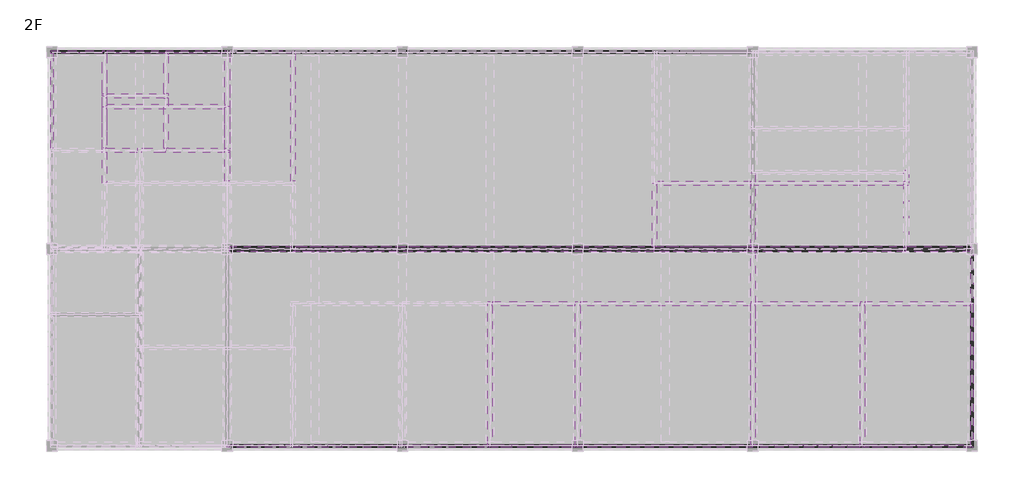
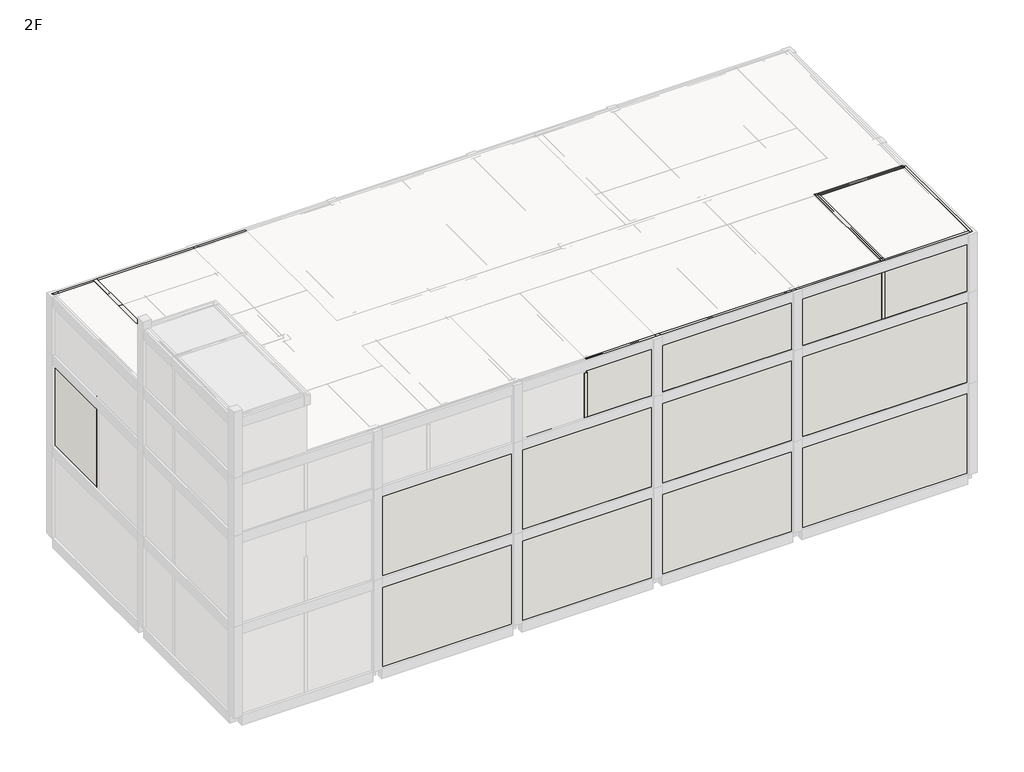
# One storey, part 2 of 7: 53 walls.
"""IFC4 building model written with IfcOpenShell, lengths in millimetres."""

from ifc_helpers import new_model, si_unit, frame, origin, place, context, project, spatial, polyline, outline, extrude, faceted_brep, element, save

model = new_model("IFC4")

# Units and contexts
model_context = context("Model", 3, world=origin())
ifc_project = project(units=[si_unit("LENGTHUNIT", "METRE", prefix="MILLI")], contexts=[model_context])

# Site, building, storey
site = spatial("IfcSite", under=ifc_project)
building = spatial("IfcBuilding", under=site)
storey = spatial("IfcBuildingStorey", under=building, Name="2F", Elevation=3500.0)

# Walls
placement = place(None, origin())
element("IfcWall", 1, ObjectType="WA211_Exterior-Cement Brick-90mm", at=placement, inside=storey, context=model_context, shape_type="Brep", body=[
    faceted_brep([(45402.6521483, 181866.8614395, 3500.0), (45516.6521483, 181866.8614395, 3500.0), (77352.6521483, 181866.8614395, 3500.0), (77352.6521483, 181866.8614395, 9000.0), (45516.6521483, 181866.8614395, 9000.0), (45402.6521483, 181866.8614395, 9000.0), (45402.6521483, 181980.8614395, 3500.0), (45402.6521483, 181980.8614395, 9000.0), (77352.6521483, 181980.8614395, 9000.0), (77352.6521483, 181980.8614395, 3500.0)], [[[0, 1, 2, 3, 4, 5]], [[6, 7, 8, 9]], [[2, 1, 0, 6, 9]], [[5, 4, 3, 8, 7]], [[0, 5, 7, 6]], [[3, 2, 9, 8]]]),
])
element("IfcWall", 2, ObjectType="WA211_Exterior-Cement Brick-90mm", at=placement, inside=storey, context=model_context, shape_type="SweptSolid", body=[
    extrude(outline(polyline([(53566.6521483, 163980.8614395), (87402.6521483, 163980.8614395), (87402.6521483, 163866.8614395), (53566.6521483, 163866.8614395), (53566.6521483, 163980.8614395)])), frame((0.0, 0.0, 3500.0), z_axis=(0.0, 0.0, 1.0), x_axis=(1.0, 0.0, 0.0)), (0.0, 0.0, 1.0), 5500.0),
])
element("IfcWall", 3, ObjectType="WA211_Exterior-Cement Brick-90mm", at=placement, inside=storey, context=model_context, shape_type="Brep", body=[
    faceted_brep([(87402.6521483, 172923.8614395, 3500.0), (87402.6521483, 172816.8614395, 3500.0), (87402.6521483, 163980.8614395, 3500.0), (87402.6521483, 163866.8614395, 3500.0), (87402.6521483, 163866.8614395, 9000.0), (87402.6521483, 163980.8614395, 9000.0), (87402.6521483, 172816.8614395, 9000.0), (87402.6521483, 172923.8614395, 9000.0), (87516.6521483, 172923.8614395, 3500.0), (87516.6521483, 172923.8614395, 9000.0), (87516.6521483, 163866.8614395, 9000.0), (87516.6521483, 163866.8614395, 3500.0)], [[[0, 1, 2, 3, 4, 5, 6, 7]], [[8, 9, 10, 11]], [[3, 2, 1, 0, 8, 11]], [[7, 6, 5, 4, 10, 9]], [[0, 7, 9, 8]], [[4, 3, 11, 10]]]),
])
element("IfcWall", 4, ObjectType="WA211_Exterior-Cement Brick-90mm", at=placement, inside=storey, context=model_context, shape_type="Brep", body=[
    faceted_brep([(77459.6521483, 163980.8614395, 9000.0), (77352.6521483, 163980.8614395, 9000.0), (53566.6521483, 163980.8614395, 9000.0), (53566.6521483, 163980.8614395, 12000.0), (53459.6521483, 163980.8614395, 12000.0), (53459.6521483, 163980.8614395, 14500.0), (77352.6521483, 163980.8614395, 14500.0), (77459.6521483, 163980.8614395, 14500.0), (77459.6521483, 163866.8614395, 9000.0), (77459.6521483, 163866.8614395, 14500.0), (53459.6521483, 163866.8614395, 14500.0), (53459.6521483, 163866.8614395, 12000.0), (53566.6521483, 163866.8614395, 12000.0), (53566.6521483, 163866.8614395, 9000.0)], [[[0, 1, 2, 3, 4, 5, 6, 7]], [[8, 9, 10, 11, 12, 13]], [[2, 1, 0, 8, 13]], [[7, 6, 5, 10, 9]], [[0, 7, 9, 8]], [[5, 4, 11, 10]], [[11, 4, 3, 12]], [[3, 2, 13, 12]]]),
])
element("IfcWall", 5, ObjectType="WA211_Exterior-Cement Brick-90mm", at=placement, inside=storey, context=model_context, shape_type="Brep", body=[
    faceted_brep([(87402.6521483, 163980.8614395, 9000.0), (77566.6521483, 163980.8614395, 9000.0), (77459.6521483, 163980.8614395, 9000.0), (77459.6521483, 163980.8614395, 14500.0), (77566.6521483, 163980.8614395, 14500.0), (87402.6521483, 163980.8614395, 14500.0), (87402.6521483, 163866.8614395, 9000.0), (87402.6521483, 163866.8614395, 14500.0), (77459.6521483, 163866.8614395, 14500.0), (77459.6521483, 163866.8614395, 9000.0)], [[[0, 1, 2, 3, 4, 5]], [[6, 7, 8, 9]], [[2, 1, 0, 6, 9]], [[3, 2, 9, 8]], [[5, 4, 3, 8, 7]], [[0, 5, 7, 6]]]),
])
element("IfcWall", 6, ObjectType="WA211_Exterior-Cement Brick-90mm", at=placement, inside=storey, context=model_context, shape_type="Brep", body=[
    faceted_brep([(87402.6521483, 172923.8614395, 9000.0), (87402.6521483, 172816.8614395, 9000.0), (87402.6521483, 163980.8614395, 9000.0), (87402.6521483, 163866.8614395, 9000.0), (87402.6521483, 163866.8614395, 14500.0), (87402.6521483, 163980.8614395, 14500.0), (87402.6521483, 172816.8614395, 14500.0), (87402.6521483, 172923.8614395, 14500.0), (87516.6521483, 172923.8614395, 9000.0), (87516.6521483, 172923.8614395, 14500.0), (87516.6521483, 163866.8614395, 14500.0), (87516.6521483, 163866.8614395, 9000.0)], [[[0, 1, 2, 3, 4, 5, 6, 7]], [[8, 9, 10, 11]], [[3, 2, 1, 0, 8, 11]], [[7, 6, 5, 4, 10, 9]], [[0, 7, 9, 8]], [[4, 3, 11, 10]]]),
])
element("IfcWall", 7, ObjectType="WA211_Exterior-Cement Brick-90mm", at=placement, inside=storey, context=model_context, shape_type="SweptSolid", body=[
    extrude(outline(polyline([(45516.6521483, 181866.8614395), (45516.6521483, 177530.8614395), (45402.6521483, 177530.8614395), (45402.6521483, 181866.8614395), (45516.6521483, 181866.8614395)])), frame((0.0, 0.0, 9000.0), z_axis=(0.0, 0.0, 1.0), x_axis=(1.0, 0.0, 0.0)), (0.0, 0.0, 1.0), 5500.0),
])
element("IfcWall", 8, ObjectType="WA211_Exterior-Cement Brick-90mm", at=placement, inside=storey, context=model_context, shape_type="Brep", body=[
    faceted_brep([(45402.6521483, 181866.8614395, 9000.0), (45516.6521483, 181866.8614395, 9000.0), (47752.6521483, 181866.8614395, 9000.0), (47752.6521483, 181866.8614395, 14500.0), (45516.6521483, 181866.8614395, 14500.0), (45402.6521483, 181866.8614395, 14500.0), (45402.6521483, 181980.8614395, 9000.0), (45402.6521483, 181980.8614395, 14500.0), (47752.6521483, 181980.8614395, 14500.0), (47752.6521483, 181980.8614395, 9000.0)], [[[0, 1, 2, 3, 4, 5]], [[6, 7, 8, 9]], [[2, 1, 0, 6, 9]], [[5, 4, 3, 8, 7]], [[0, 5, 7, 6]], [[3, 2, 9, 8]]]),
])
element("IfcWall", 9, ObjectType="WA211_Exterior-Cement Brick-90mm", at=placement, inside=storey, context=model_context, shape_type="Brep", body=[
    faceted_brep([(50659.6521483, 181866.8614395, 14500.0), (50659.6521483, 181866.8614395, 9000.0), (50766.6521483, 181866.8614395, 9000.0), (53352.6521483, 181866.8614395, 9000.0), (53352.6521483, 181866.8614395, 12400.0), (53459.6521483, 181866.8614395, 12400.0), (53459.6521483, 181866.8614395, 14500.0), (50659.6521483, 181980.8614395, 9000.0), (50659.6521483, 181980.8614395, 14500.0), (53459.6521483, 181980.8614395, 14500.0), (53459.6521483, 181980.8614395, 12400.0), (53352.6521483, 181980.8614395, 12400.0), (53352.6521483, 181980.8614395, 9000.0)], [[[0, 1, 2, 3, 4, 5, 6]], [[7, 8, 9, 10, 11, 12]], [[3, 2, 1, 7, 12]], [[0, 6, 9, 8]], [[6, 5, 10, 9]], [[10, 5, 4, 11]], [[4, 3, 12, 11]], [[0, 8, 7, 1]]]),
])
element("IfcWall", 10, ObjectType="WA211_Exterior-Cement Brick-90mm", at=placement, inside=storey, context=model_context, shape_type="Brep", body=[
    faceted_brep([(47966.6521483, 181866.8614395, 9000.0), (50552.6521483, 181866.8614395, 9000.0), (50659.6521483, 181866.8614395, 9000.0), (50659.6521483, 181866.8614395, 14500.0), (47966.6521483, 181866.8614395, 14500.0), (47966.6521483, 181980.8614395, 9000.0), (47966.6521483, 181980.8614395, 14500.0), (50659.6521483, 181980.8614395, 14500.0), (50659.6521483, 181980.8614395, 9000.0)], [[[0, 1, 2, 3, 4]], [[5, 6, 7, 8]], [[2, 1, 0, 5, 8]], [[4, 3, 7, 6]], [[0, 4, 6, 5]], [[2, 8, 7, 3]]]),
])
element("IfcWall", 11, ObjectType="WA211_Exterior-Cement Brick-90mm", at=placement, inside=storey, context=model_context, shape_type="SweptSolid", body=[
    extrude(outline(polyline([(14500.0, 69352.6521483), (17200.0, 69352.6521483), (17200.0, 69459.6521483), (18000.0, 69459.6521483), (18000.0, 65459.6521483), (17200.0, 65459.6521483), (17200.0, 65566.6521483), (14500.0, 65566.6521483), (14500.0, 69352.6521483)])), frame((0.0, 163866.8614395, 0.0), z_axis=(0.0, 1.0, 0.0), x_axis=(0.0, 0.0, 1.0)), (0.0, 0.0, 1.0), 114.0),
])
element("IfcWall", 12, ObjectType="WA211_Exterior-Cement Brick-90mm", at=placement, inside=storey, context=model_context, shape_type="Brep", body=[
    faceted_brep([(77459.6521483, 163980.8614395, 18000.0), (77459.6521483, 163980.8614395, 14500.0), (77352.6521483, 163980.8614395, 14500.0), (69566.6521483, 163980.8614395, 14500.0), (69566.6521483, 163980.8614395, 17200.0), (69459.6521483, 163980.8614395, 17200.0), (69459.6521483, 163980.8614395, 18000.0), (77459.6521483, 163866.8614395, 14500.0), (77459.6521483, 163866.8614395, 18000.0), (69459.6521483, 163866.8614395, 18000.0), (69459.6521483, 163866.8614395, 17200.0), (69566.6521483, 163866.8614395, 17200.0), (69566.6521483, 163866.8614395, 14500.0)], [[[0, 1, 2, 3, 4, 5, 6]], [[7, 8, 9, 10, 11, 12]], [[3, 2, 1, 7, 12]], [[0, 6, 9, 8]], [[6, 5, 10, 9]], [[10, 5, 4, 11]], [[4, 3, 12, 11]], [[0, 8, 7, 1]]]),
])
element("IfcWall", 13, ObjectType="WA211_Exterior-Cement Brick-90mm", at=placement, inside=storey, context=model_context, shape_type="Brep", body=[
    faceted_brep([(82352.6521483, 163980.8614395, 14500.0), (77566.6521483, 163980.8614395, 14500.0), (77459.6521483, 163980.8614395, 14500.0), (77459.6521483, 163980.8614395, 18000.0), (82352.6521483, 163980.8614395, 18000.0), (82352.6521483, 163866.8614395, 14500.0), (82352.6521483, 163866.8614395, 18000.0), (77459.6521483, 163866.8614395, 18000.0), (77459.6521483, 163866.8614395, 14500.0)], [[[0, 1, 2, 3, 4]], [[5, 6, 7, 8]], [[2, 1, 0, 5, 8]], [[4, 3, 7, 6]], [[2, 8, 7, 3]], [[0, 4, 6, 5]]]),
])
element("IfcWall", 14, ObjectType="WA211_Exterior-Cement Brick-90mm", at=placement, inside=storey, context=model_context, shape_type="SweptSolid", body=[
    extrude(outline(polyline([(82566.6521483, 163980.8614395), (87402.6521483, 163980.8614395), (87402.6521483, 163866.8614395), (82566.6521483, 163866.8614395), (82566.6521483, 163980.8614395)])), frame((0.0, 0.0, 14500.0), z_axis=(0.0, 0.0, 1.0), x_axis=(1.0, 0.0, 0.0)), (0.0, 0.0, 1.0), 3500.0),
])
element("IfcWall", 15, ObjectType="WA211_Exterior-Cement Brick-90mm", at=placement, inside=storey, context=model_context, shape_type="Brep", body=[
    faceted_brep([(87402.6521483, 170423.8614395, 14500.0), (87402.6521483, 170316.8614395, 14500.0), (87402.6521483, 163980.8614395, 14500.0), (87402.6521483, 163866.8614395, 14500.0), (87402.6521483, 163866.8614395, 18000.0), (87402.6521483, 163980.8614395, 18000.0), (87402.6521483, 170316.8614395, 18000.0), (87402.6521483, 170423.8614395, 18000.0), (87516.6521483, 170423.8614395, 14500.0), (87516.6521483, 170423.8614395, 18000.0), (87516.6521483, 163866.8614395, 18000.0), (87516.6521483, 163866.8614395, 14500.0)], [[[0, 1, 2, 3, 4, 5, 6, 7]], [[8, 9, 10, 11]], [[3, 2, 1, 0, 8, 11]], [[7, 6, 5, 4, 10, 9]], [[0, 7, 9, 8]], [[4, 3, 11, 10]]]),
])
element("IfcWall", 16, ObjectType="WA211_Exterior-Cement Brick-90mm", at=placement, inside=storey, context=model_context, shape_type="SweptSolid", body=[
    extrude(outline(polyline([(14500.0, 47966.6521483), (14500.0, 53352.6521483), (17200.0, 53352.6521483), (17200.0, 53459.6521483), (18000.0, 53459.6521483), (18000.0, 47966.6521483), (14500.0, 47966.6521483)])), frame((0.0, 181866.8614395, 0.0), z_axis=(0.0, 1.0, 0.0), x_axis=(0.0, 0.0, 1.0)), (0.0, 0.0, 1.0), 114.0),
])
element("IfcWall", 17, ObjectType="WA211_Exterior-Cement Brick-90mm", at=placement, inside=storey, context=model_context, shape_type="SweptSolid", body=[
    extrude(outline(polyline([(14500.0, 53566.6521483), (14500.0, 56352.6521483), (17200.0, 56352.6521483), (17200.0, 56459.6521483), (18000.0, 56459.6521483), (18000.0, 53459.6521483), (17200.0, 53459.6521483), (17200.0, 53566.6521483), (14500.0, 53566.6521483)])), frame((0.0, 181866.8614395, 0.0), z_axis=(0.0, 1.0, 0.0), x_axis=(0.0, 0.0, 1.0)), (0.0, 0.0, 1.0), 114.0),
])
element("IfcWall", 18, ObjectType="WA211_Exterior-Cement Brick-90mm", at=placement, inside=storey, context=model_context, shape_type="Brep", body=[
    faceted_brep([(45402.6521483, 181866.8614395, 14500.0), (45516.6521483, 181866.8614395, 14500.0), (47752.6521483, 181866.8614395, 14500.0), (47752.6521483, 181866.8614395, 18000.0), (45516.6521483, 181866.8614395, 18000.0), (45402.6521483, 181866.8614395, 18000.0), (45402.6521483, 181980.8614395, 14500.0), (45402.6521483, 181980.8614395, 18000.0), (47752.6521483, 181980.8614395, 18000.0), (47752.6521483, 181980.8614395, 14500.0)], [[[0, 1, 2, 3, 4, 5]], [[6, 7, 8, 9]], [[2, 1, 0, 6, 9]], [[5, 4, 3, 8, 7]], [[3, 2, 9, 8]], [[0, 5, 7, 6]]]),
])
element("IfcWall", 19, ObjectType="WA221_Interior-Cement Block-190mm", at=placement, inside=storey, context=model_context, shape_type="SweptSolid", body=[
    extrude(outline(polyline([(53566.6521483, 173030.8614395), (77352.6521483, 173030.8614395), (77352.6521483, 172816.8614395), (53566.6521483, 172816.8614395), (53566.6521483, 173030.8614395)])), frame((0.0, 0.0, 3500.0), z_axis=(0.0, 0.0, 1.0), x_axis=(1.0, 0.0, 0.0)), (0.0, 0.0, 1.0), 5500.0),
])
element("IfcWall", 20, ObjectType="WA221_Interior-Cement Block-190mm", at=placement, inside=storey, context=model_context, shape_type="Brep", body=[
    faceted_brep([(77566.6521483, 172816.8614395, 3500.0), (87402.6521483, 172816.8614395, 3500.0), (87402.6521483, 172816.8614395, 9000.0), (77566.6521483, 172816.8614395, 9000.0), (77566.6521483, 173030.8614395, 3500.0), (77566.6521483, 173030.8614395, 9000.0), (87402.6521483, 173030.8614395, 9000.0), (87402.6521483, 173030.8614395, 3500.0), (87402.6521483, 172923.8614395, 3500.0), (87402.6521483, 172923.8614395, 9000.0)], [[[0, 1, 2, 3]], [[4, 5, 6, 7]], [[1, 0, 4, 7, 8]], [[3, 2, 9, 6, 5]], [[0, 3, 5, 4]], [[2, 1, 8, 7, 6, 9]]]),
])
element("IfcWall", 21, ObjectType="WA221_Interior-Cement Block-190mm", at=placement, inside=storey, context=model_context, shape_type="Brep", body=[
    faceted_brep([(77459.6521483, 173030.8614395, 9000.0), (77352.6521483, 173030.8614395, 9000.0), (53566.6521483, 173030.8614395, 9000.0), (53566.6521483, 173030.8614395, 12400.0), (77352.6521483, 173030.8614395, 12400.0), (77459.6521483, 173030.8614395, 12400.0), (77459.6521483, 172816.8614395, 9000.0), (77459.6521483, 172816.8614395, 12400.0), (77352.6521483, 172816.8614395, 12400.0), (53566.6521483, 172816.8614395, 12400.0), (53566.6521483, 172816.8614395, 12000.0), (53566.6521483, 172816.8614395, 9000.0), (77352.6521483, 172816.8614395, 9000.0), (53566.6521483, 172923.8614395, 9000.0)], [[[0, 1, 2, 3, 4, 5]], [[6, 7, 8, 9, 10, 11, 12]], [[2, 1, 0, 6, 12, 11, 13]], [[5, 4, 3, 9, 8, 7]], [[0, 5, 7, 6]], [[2, 13, 11, 10, 9, 3]]]),
])
element("IfcWall", 22, ObjectType="WA221_Interior-Cement Block-190mm", at=placement, inside=storey, context=model_context, shape_type="Brep", body=[
    faceted_brep([(77352.6521483, 176316.8614395, 9000.0), (77352.6521483, 173030.8614395, 9000.0), (77352.6521483, 173030.8614395, 12400.0), (77352.6521483, 176423.8614395, 12400.0), (77352.6521483, 176423.8614395, 11700.0), (77352.6521483, 176316.8614395, 11700.0), (77566.6521483, 176316.8614395, 9000.0), (77566.6521483, 176316.8614395, 11700.0), (77566.6521483, 176423.8614395, 11700.0), (77566.6521483, 176423.8614395, 12400.0), (77566.6521483, 173030.8614395, 12400.0), (77566.6521483, 173030.8614395, 9000.0), (77459.6521483, 173030.8614395, 9000.0), (77459.6521483, 173030.8614395, 12400.0)], [[[0, 1, 2, 3, 4, 5]], [[6, 7, 8, 9, 10, 11]], [[1, 0, 6, 11, 12]], [[3, 2, 13, 10, 9]], [[2, 1, 12, 11, 10, 13]], [[4, 3, 9, 8]], [[4, 8, 7, 5]], [[0, 5, 7, 6]]]),
])
element("IfcWall", 23, ObjectType="WA221_Interior-Cement Block-190mm", at=placement, inside=storey, context=model_context, shape_type="Brep", body=[
    faceted_brep([(53566.6521483, 177530.8614395, 9000.0), (53566.6521483, 181866.8614395, 9000.0), (53566.6521483, 181980.8614395, 9000.0), (53566.6521483, 181980.8614395, 12400.0), (53566.6521483, 181866.8614395, 12400.0), (53566.6521483, 177423.8614395, 12400.0), (53566.6521483, 177423.8614395, 11700.0), (53566.6521483, 177530.8614395, 11700.0), (53352.6521483, 177530.8614395, 9000.0), (53352.6521483, 177530.8614395, 11700.0), (53352.6521483, 177423.8614395, 11700.0), (53352.6521483, 177423.8614395, 12400.0), (53352.6521483, 181866.8614395, 12400.0), (53352.6521483, 181980.8614395, 12400.0), (53352.6521483, 181980.8614395, 9000.0), (53352.6521483, 181866.8614395, 9000.0), (53459.6521483, 181980.8614395, 12400.0)], [[[0, 1, 2, 3, 4, 5, 6, 7]], [[8, 9, 10, 11, 12, 13, 14, 15]], [[2, 1, 0, 8, 15, 14]], [[5, 4, 3, 16, 13, 12, 11]], [[3, 2, 14, 13, 16]], [[6, 5, 11, 10]], [[6, 10, 9, 7]], [[0, 7, 9, 8]]]),
])
element("IfcWall", 24, ObjectType="WA221_Interior-Cement Block-190mm", at=placement, inside=storey, context=model_context, shape_type="Brep", body=[
    faceted_brep([(77566.6521483, 163980.8614395, 9000.0), (77566.6521483, 172816.8614395, 9000.0), (77566.6521483, 172816.8614395, 14500.0), (77566.6521483, 163980.8614395, 14500.0), (77352.6521483, 163980.8614395, 9000.0), (77352.6521483, 163980.8614395, 14500.0), (77352.6521483, 172816.8614395, 14500.0), (77352.6521483, 172816.8614395, 12400.0), (77352.6521483, 172816.8614395, 9000.0), (77459.6521483, 163980.8614395, 9000.0), (77459.6521483, 172816.8614395, 9000.0), (77459.6521483, 163980.8614395, 14500.0)], [[[0, 1, 2, 3]], [[4, 5, 6, 7, 8]], [[1, 0, 9, 4, 8, 10]], [[3, 2, 6, 5, 11]], [[1, 10, 8, 7, 6, 2]], [[0, 3, 11, 5, 4, 9]]]),
])
element("IfcWall", 25, ObjectType="WA221_Interior-Cement Block-190mm", at=placement, inside=storey, context=model_context, shape_type="Brep", body=[
    faceted_brep([(77459.6521483, 172816.8614395, 9000.0), (77566.6521483, 172816.8614395, 9000.0), (84459.6521483, 172816.8614395, 9000.0), (84459.6521483, 172816.8614395, 14500.0), (77566.6521483, 172816.8614395, 14500.0), (77352.6521483, 172816.8614395, 14500.0), (77352.6521483, 172816.8614395, 12400.0), (77459.6521483, 172816.8614395, 12400.0), (77459.6521483, 173030.8614395, 9000.0), (77459.6521483, 173030.8614395, 12400.0), (77352.6521483, 173030.8614395, 12400.0), (77352.6521483, 173030.8614395, 14500.0), (84459.6521483, 173030.8614395, 14500.0), (84459.6521483, 173030.8614395, 9000.0), (84352.6521483, 173030.8614395, 9000.0), (77566.6521483, 173030.8614395, 9000.0)], [[[0, 1, 2, 3, 4, 5, 6, 7]], [[8, 9, 10, 11, 12, 13, 14, 15]], [[2, 1, 0, 8, 15, 14, 13]], [[5, 4, 3, 12, 11]], [[0, 7, 9, 8]], [[6, 10, 9, 7]], [[6, 5, 11, 10]], [[2, 13, 12, 3]]]),
])
element("IfcWall", 26, ObjectType="WA221_Interior-Cement Block-190mm", at=placement, inside=storey, context=model_context, shape_type="Brep", body=[
    faceted_brep([(84459.6521483, 172816.8614395, 14500.0), (84459.6521483, 172816.8614395, 9000.0), (87402.6521483, 172816.8614395, 9000.0), (87402.6521483, 172816.8614395, 14500.0), (84459.6521483, 173030.8614395, 9000.0), (84459.6521483, 173030.8614395, 14500.0), (87402.6521483, 173030.8614395, 14500.0), (87402.6521483, 173030.8614395, 9000.0), (84566.6521483, 173030.8614395, 9000.0), (87402.6521483, 172923.8614395, 9000.0), (87402.6521483, 172923.8614395, 14500.0)], [[[0, 1, 2, 3]], [[4, 5, 6, 7, 8]], [[2, 1, 4, 8, 7, 9]], [[0, 3, 10, 6, 5]], [[3, 2, 9, 7, 6, 10]], [[0, 5, 4, 1]]]),
])
element("IfcWall", 27, ObjectType="WA221_Interior-Cement Block-190mm", at=placement, inside=storey, context=model_context, shape_type="Brep", body=[
    faceted_brep([(84352.6521483, 176530.8614395, 9000.0), (84352.6521483, 176316.8614395, 9000.0), (84352.6521483, 173030.8614395, 9000.0), (84352.6521483, 173030.8614395, 11700.0), (84352.6521483, 176316.8614395, 11700.0), (84352.6521483, 176530.8614395, 11700.0), (84566.6521483, 176530.8614395, 9000.0), (84566.6521483, 176530.8614395, 11700.0), (84566.6521483, 173030.8614395, 11700.0), (84566.6521483, 173030.8614395, 9000.0), (84459.6521483, 173030.8614395, 9000.0)], [[[0, 1, 2, 3, 4, 5]], [[6, 7, 8, 9]], [[2, 1, 0, 6, 9, 10]], [[5, 4, 3, 8, 7]], [[0, 5, 7, 6]], [[3, 2, 10, 9, 8]]]),
])
element("IfcWall", 28, ObjectType="WA221_Interior-Cement Block-190mm", at=placement, inside=storey, context=model_context, shape_type="Brep", body=[
    faceted_brep([(47752.6521483, 181980.8614395, 9000.0), (47752.6521483, 181866.8614395, 9000.0), (47752.6521483, 180030.8614395, 9000.0), (47752.6521483, 180030.8614395, 11700.0), (47752.6521483, 179923.8614395, 11700.0), (47752.6521483, 179923.8614395, 14500.0), (47752.6521483, 181866.8614395, 14500.0), (47752.6521483, 181980.8614395, 14500.0), (47966.6521483, 181980.8614395, 9000.0), (47966.6521483, 181980.8614395, 14500.0), (47966.6521483, 181866.8614395, 14500.0), (47966.6521483, 179923.8614395, 14500.0), (47966.6521483, 179923.8614395, 11700.0), (47966.6521483, 180030.8614395, 11700.0), (47966.6521483, 180030.8614395, 9000.0), (47966.6521483, 181866.8614395, 9000.0)], [[[0, 1, 2, 3, 4, 5, 6, 7]], [[8, 9, 10, 11, 12, 13, 14, 15]], [[2, 1, 0, 8, 15, 14]], [[7, 6, 5, 11, 10, 9]], [[0, 7, 9, 8]], [[5, 4, 12, 11]], [[12, 4, 3, 13]], [[3, 2, 14, 13]]]),
])
element("IfcWall", 29, ObjectType="WA221_Interior-Cement Block-190mm", at=placement, inside=storey, context=model_context, shape_type="Brep", body=[
    faceted_brep([(47752.6521483, 179816.8614395, 9000.0), (47752.6521483, 177530.8614395, 9000.0), (47752.6521483, 177530.8614395, 14500.0), (47752.6521483, 179923.8614395, 14500.0), (47752.6521483, 179923.8614395, 11700.0), (47752.6521483, 179816.8614395, 11700.0), (47966.6521483, 179816.8614395, 9000.0), (47966.6521483, 179816.8614395, 11700.0), (47966.6521483, 179923.8614395, 11700.0), (47966.6521483, 179923.8614395, 14500.0), (47966.6521483, 177530.8614395, 14500.0), (47966.6521483, 177530.8614395, 11700.0), (47966.6521483, 177530.8614395, 9000.0), (47859.6521483, 177530.8614395, 9000.0)], [[[0, 1, 2, 3, 4, 5]], [[6, 7, 8, 9, 10, 11, 12]], [[1, 0, 6, 12, 13]], [[3, 2, 10, 9]], [[1, 13, 12, 11, 10, 2]], [[4, 3, 9, 8]], [[4, 8, 7, 5]], [[0, 5, 7, 6]]]),
])
element("IfcWall", 30, ObjectType="WA221_Interior-Cement Block-190mm", at=placement, inside=storey, context=model_context, shape_type="Brep", body=[
    faceted_brep([(49352.6521483, 177530.8614395, 9000.0), (47966.6521483, 177530.8614395, 9000.0), (47859.6521483, 177530.8614395, 9000.0), (47859.6521483, 177530.8614395, 11700.0), (47966.6521483, 177530.8614395, 11700.0), (49352.6521483, 177530.8614395, 11700.0), (49352.6521483, 177316.8614395, 9000.0), (49352.6521483, 177316.8614395, 11700.0), (47966.6521483, 177316.8614395, 11700.0), (47859.6521483, 177316.8614395, 11700.0), (47859.6521483, 177316.8614395, 9000.0)], [[[0, 1, 2, 3, 4, 5]], [[6, 7, 8, 9, 10]], [[2, 1, 0, 6, 10]], [[3, 2, 10, 9]], [[5, 4, 3, 9, 8, 7]], [[0, 5, 7, 6]]]),
])
element("IfcWall", 31, ObjectType="WA221_Interior-Cement Block-190mm", at=placement, inside=storey, context=model_context, shape_type="Brep", body=[
    faceted_brep([(50552.6521483, 181866.8614395, 9000.0), (50552.6521483, 180030.8614395, 9000.0), (50552.6521483, 180030.8614395, 11700.0), (50552.6521483, 181866.8614395, 11700.0), (50766.6521483, 181866.8614395, 9000.0), (50766.6521483, 181866.8614395, 11700.0), (50766.6521483, 180030.8614395, 11700.0), (50766.6521483, 180030.8614395, 9000.0), (50659.6521483, 181866.8614395, 9000.0)], [[[0, 1, 2, 3]], [[4, 5, 6, 7]], [[1, 0, 8, 4, 7]], [[3, 2, 6, 5]], [[0, 3, 5, 4, 8]], [[2, 1, 7, 6]]]),
])
element("IfcWall", 32, ObjectType="WA221_Interior-Cement Block-190mm", at=placement, inside=storey, context=model_context, shape_type="Brep", body=[
    faceted_brep([(50766.6521483, 177530.8614395, 9000.0), (50766.6521483, 179816.8614395, 9000.0), (50766.6521483, 179816.8614395, 11700.0), (50766.6521483, 177530.8614395, 11700.0), (50552.6521483, 177530.8614395, 9000.0), (50552.6521483, 177530.8614395, 11700.0), (50552.6521483, 179816.8614395, 11700.0), (50552.6521483, 179816.8614395, 9000.0), (50659.6521483, 177530.8614395, 9000.0), (50659.6521483, 177530.8614395, 11700.0)], [[[0, 1, 2, 3]], [[4, 5, 6, 7]], [[1, 0, 8, 4, 7]], [[3, 2, 6, 5, 9]], [[0, 3, 9, 5, 4, 8]], [[2, 1, 7, 6]]]),
])
element("IfcWall", 33, ObjectType="WA221_Interior-Cement Block-190mm", at=placement, inside=storey, context=model_context, shape_type="Brep", body=[
    faceted_brep([(50659.6521483, 177316.8614395, 9000.0), (53352.6521483, 177316.8614395, 9000.0), (53566.6521483, 177316.8614395, 9000.0), (53566.6521483, 177316.8614395, 11700.0), (53352.6521483, 177316.8614395, 11700.0), (50659.6521483, 177316.8614395, 11700.0), (50659.6521483, 177530.8614395, 9000.0), (50659.6521483, 177530.8614395, 11700.0), (50766.6521483, 177530.8614395, 11700.0), (53352.6521483, 177530.8614395, 11700.0), (53566.6521483, 177530.8614395, 11700.0), (53566.6521483, 177530.8614395, 9000.0), (53352.6521483, 177530.8614395, 9000.0), (50766.6521483, 177530.8614395, 9000.0), (53566.6521483, 177423.8614395, 11700.0)], [[[0, 1, 2, 3, 4, 5]], [[6, 7, 8, 9, 10, 11, 12, 13]], [[2, 1, 0, 6, 13, 12, 11]], [[5, 4, 3, 14, 10, 9, 8, 7]], [[0, 5, 7, 6]], [[3, 2, 11, 10, 14]]]),
])
element("IfcWall", 34, ObjectType="WA221_Interior-Cement Block-190mm", at=placement, inside=storey, context=model_context, shape_type="Brep", body=[
    faceted_brep([(50766.6521483, 180030.8614395, 9000.0), (50552.6521483, 180030.8614395, 9000.0), (47966.6521483, 180030.8614395, 9000.0), (47752.6521483, 180030.8614395, 9000.0), (47752.6521483, 180030.8614395, 11700.0), (47966.6521483, 180030.8614395, 11700.0), (50552.6521483, 180030.8614395, 11700.0), (50766.6521483, 180030.8614395, 11700.0), (50766.6521483, 179816.8614395, 9000.0), (50766.6521483, 179816.8614395, 11700.0), (50552.6521483, 179816.8614395, 11700.0), (47966.6521483, 179816.8614395, 11700.0), (47752.6521483, 179816.8614395, 11700.0), (47752.6521483, 179816.8614395, 9000.0), (47966.6521483, 179816.8614395, 9000.0), (50552.6521483, 179816.8614395, 9000.0), (47752.6521483, 179923.8614395, 11700.0)], [[[0, 1, 2, 3, 4, 5, 6, 7]], [[8, 9, 10, 11, 12, 13, 14, 15]], [[3, 2, 1, 0, 8, 15, 14, 13]], [[7, 6, 5, 4, 16, 12, 11, 10, 9]], [[0, 7, 9, 8]], [[4, 3, 13, 12, 16]]]),
])
element("IfcWall", 35, ObjectType="WA221_Interior-Cement Block-190mm", at=placement, inside=storey, context=model_context, shape_type="Brep", body=[
    faceted_brep([(50659.6521483, 177530.8614395, 9000.0), (50552.6521483, 177530.8614395, 9000.0), (49566.6521483, 177530.8614395, 9000.0), (49566.6521483, 177530.8614395, 11700.0), (50552.6521483, 177530.8614395, 11700.0), (50659.6521483, 177530.8614395, 11700.0), (50659.6521483, 177316.8614395, 9000.0), (50659.6521483, 177316.8614395, 11700.0), (49566.6521483, 177316.8614395, 11700.0), (49566.6521483, 177316.8614395, 9000.0)], [[[0, 1, 2, 3, 4, 5]], [[6, 7, 8, 9]], [[2, 1, 0, 6, 9]], [[5, 4, 3, 8, 7]], [[0, 5, 7, 6]], [[3, 2, 9, 8]]]),
])
element("IfcWall", 36, ObjectType="WA221_Interior-Cement Block-190mm", at=placement, inside=storey, context=model_context, shape_type="Brep", body=[
    faceted_brep([(65352.6521483, 170530.8614395, 14500.0), (65352.6521483, 170316.8614395, 14500.0), (65352.6521483, 163980.8614395, 14500.0), (65352.6521483, 163866.8614395, 14500.0), (65352.6521483, 163866.8614395, 17200.0), (65352.6521483, 163980.8614395, 17200.0), (65352.6521483, 170316.8614395, 17200.0), (65352.6521483, 170530.8614395, 17200.0), (65566.6521483, 170530.8614395, 14500.0), (65566.6521483, 170530.8614395, 17200.0), (65566.6521483, 170316.8614395, 17200.0), (65566.6521483, 163980.8614395, 17200.0), (65566.6521483, 163866.8614395, 17200.0), (65566.6521483, 163866.8614395, 14500.0), (65566.6521483, 163980.8614395, 14500.0), (65566.6521483, 170316.8614395, 14500.0), (65459.6521483, 163866.8614395, 17200.0)], [[[0, 1, 2, 3, 4, 5, 6, 7]], [[8, 9, 10, 11, 12, 13, 14, 15]], [[3, 2, 1, 0, 8, 15, 14, 13]], [[7, 6, 5, 4, 16, 12, 11, 10, 9]], [[4, 3, 13, 12, 16]], [[0, 7, 9, 8]]]),
])
element("IfcWall", 37, ObjectType="WA221_Interior-Cement Block-190mm", at=placement, inside=storey, context=model_context, shape_type="Brep", body=[
    faceted_brep([(69566.6521483, 163866.8614395, 14500.0), (69566.6521483, 163980.8614395, 14500.0), (69566.6521483, 170316.8614395, 14500.0), (69566.6521483, 170530.8614395, 14500.0), (69566.6521483, 170530.8614395, 17200.0), (69566.6521483, 170316.8614395, 17200.0), (69566.6521483, 163980.8614395, 17200.0), (69566.6521483, 163866.8614395, 17200.0), (69352.6521483, 163866.8614395, 14500.0), (69352.6521483, 163866.8614395, 17200.0), (69352.6521483, 163980.8614395, 17200.0), (69352.6521483, 170316.8614395, 17200.0), (69352.6521483, 170530.8614395, 17200.0), (69352.6521483, 170530.8614395, 14500.0), (69352.6521483, 170316.8614395, 14500.0), (69352.6521483, 163980.8614395, 14500.0), (69459.6521483, 163866.8614395, 17200.0)], [[[0, 1, 2, 3, 4, 5, 6, 7]], [[8, 9, 10, 11, 12, 13, 14, 15]], [[3, 2, 1, 0, 8, 15, 14, 13]], [[7, 6, 5, 4, 12, 11, 10, 9, 16]], [[4, 3, 13, 12]], [[0, 7, 16, 9, 8]]]),
])
element("IfcWall", 38, ObjectType="WA221_Interior-Cement Block-190mm", at=placement, inside=storey, context=model_context, shape_type="SweptSolid", body=[
    extrude(outline(polyline([(65566.6521483, 170530.8614395), (69352.6521483, 170530.8614395), (69352.6521483, 170316.8614395), (65566.6521483, 170316.8614395), (65566.6521483, 170530.8614395)])), frame((0.0, 0.0, 14500.0), z_axis=(0.0, 0.0, 1.0), x_axis=(1.0, 0.0, 0.0)), (0.0, 0.0, 1.0), 2700.0),
])
element("IfcWall", 39, ObjectType="WA221_Interior-Cement Block-190mm", at=placement, inside=storey, context=model_context, shape_type="Brep", body=[
    faceted_brep([(84566.6521483, 176030.8614395, 14500.0), (84352.6521483, 176030.8614395, 14500.0), (73066.6521483, 176030.8614395, 14500.0), (73066.6521483, 176030.8614395, 17200.0), (84352.6521483, 176030.8614395, 17200.0), (84566.6521483, 176030.8614395, 17200.0), (84566.6521483, 175816.8614395, 14500.0), (84566.6521483, 175816.8614395, 17200.0), (84352.6521483, 175816.8614395, 17200.0), (73066.6521483, 175816.8614395, 17200.0), (73066.6521483, 175816.8614395, 14500.0), (84352.6521483, 175816.8614395, 14500.0), (73066.6521483, 175923.8614395, 14500.0), (73066.6521483, 175923.8614395, 17200.0)], [[[0, 1, 2, 3, 4, 5]], [[6, 7, 8, 9, 10, 11]], [[2, 1, 0, 6, 11, 10, 12]], [[5, 4, 3, 13, 9, 8, 7]], [[0, 5, 7, 6]], [[3, 2, 12, 10, 9, 13]]]),
])
element("IfcWall", 40, ObjectType="WA221_Interior-Cement Block-190mm", at=placement, inside=storey, context=model_context, shape_type="Brep", body=[
    faceted_brep([(77352.6521483, 170530.8614395, 14500.0), (77352.6521483, 170316.8614395, 14500.0), (77352.6521483, 163980.8614395, 14500.0), (77352.6521483, 163980.8614395, 17200.0), (77352.6521483, 170316.8614395, 17200.0), (77352.6521483, 170530.8614395, 17200.0), (77566.6521483, 170530.8614395, 14500.0), (77566.6521483, 170530.8614395, 17200.0), (77566.6521483, 170316.8614395, 17200.0), (77566.6521483, 163980.8614395, 17200.0), (77566.6521483, 163980.8614395, 14500.0), (77566.6521483, 170316.8614395, 14500.0), (77459.6521483, 163980.8614395, 14500.0)], [[[0, 1, 2, 3, 4, 5]], [[6, 7, 8, 9, 10, 11]], [[2, 1, 0, 6, 11, 10, 12]], [[5, 4, 3, 9, 8, 7]], [[0, 5, 7, 6]], [[3, 2, 12, 10, 9]]]),
])
element("IfcWall", 41, ObjectType="WA221_Interior-Cement Block-190mm", at=placement, inside=storey, context=model_context, shape_type="SweptSolid", body=[
    extrude(outline(polyline([(77352.6521483, 170316.8614395), (69566.6521483, 170316.8614395), (69566.6521483, 170530.8614395), (77352.6521483, 170530.8614395), (77352.6521483, 170316.8614395)])), frame((0.0, 0.0, 14500.0), z_axis=(0.0, 0.0, 1.0), x_axis=(1.0, 0.0, 0.0)), (0.0, 0.0, 1.0), 2700.0),
])
element("IfcWall", 42, ObjectType="WA221_Interior-Cement Block-190mm", at=placement, inside=storey, context=model_context, shape_type="Brep", body=[
    faceted_brep([(73066.6521483, 173030.8614395, 14500.0), (73066.6521483, 175816.8614395, 14500.0), (73066.6521483, 175923.8614395, 14500.0), (73066.6521483, 175923.8614395, 17200.0), (73066.6521483, 175816.8614395, 17200.0), (73066.6521483, 173030.8614395, 17200.0), (72852.6521483, 173030.8614395, 14500.0), (72852.6521483, 173030.8614395, 17200.0), (72852.6521483, 175923.8614395, 17200.0), (72852.6521483, 175923.8614395, 14500.0), (72959.6521483, 173030.8614395, 14500.0), (72959.6521483, 173030.8614395, 17200.0)], [[[0, 1, 2, 3, 4, 5]], [[6, 7, 8, 9]], [[2, 1, 0, 10, 6, 9]], [[3, 2, 9, 8]], [[5, 4, 3, 8, 7, 11]], [[0, 5, 11, 7, 6, 10]]]),
])
element("IfcWall", 43, ObjectType="WA221_Interior-Cement Block-190mm", at=placement, inside=storey, context=model_context, shape_type="Brep", body=[
    faceted_brep([(56352.6521483, 181980.8614395, 14500.0), (56352.6521483, 181866.8614395, 14500.0), (56352.6521483, 176030.8614395, 14500.0), (56352.6521483, 176030.8614395, 17200.0), (56352.6521483, 181866.8614395, 17200.0), (56352.6521483, 181980.8614395, 17200.0), (56566.6521483, 181980.8614395, 14500.0), (56566.6521483, 181980.8614395, 17200.0), (56566.6521483, 181866.8614395, 17200.0), (56566.6521483, 176030.8614395, 17200.0), (56566.6521483, 176030.8614395, 14500.0), (56566.6521483, 181866.8614395, 14500.0), (56459.6521483, 181980.8614395, 17200.0)], [[[0, 1, 2, 3, 4, 5]], [[6, 7, 8, 9, 10, 11]], [[2, 1, 0, 6, 11, 10]], [[5, 4, 3, 9, 8, 7, 12]], [[0, 5, 12, 7, 6]], [[3, 2, 10, 9]]]),
])
element("IfcWall", 44, ObjectType="WA221_Interior-Cement Block-190mm", at=placement, inside=storey, context=model_context, shape_type="Brep", body=[
    faceted_brep([(72959.6521483, 173030.8614395, 14500.0), (72852.6521483, 173030.8614395, 14500.0), (56566.6521483, 173030.8614395, 14500.0), (56566.6521483, 173030.8614395, 17200.0), (72852.6521483, 173030.8614395, 17200.0), (72959.6521483, 173030.8614395, 17200.0), (72959.6521483, 172816.8614395, 14500.0), (72959.6521483, 172816.8614395, 17200.0), (56566.6521483, 172816.8614395, 17200.0), (56566.6521483, 172816.8614395, 14500.0)], [[[0, 1, 2, 3, 4, 5]], [[6, 7, 8, 9]], [[2, 1, 0, 6, 9]], [[5, 4, 3, 8, 7]], [[0, 5, 7, 6]], [[3, 2, 9, 8]]]),
])
element("IfcWall", 45, ObjectType="WA221_Interior-Cement Block-190mm", at=placement, inside=storey, context=model_context, shape_type="Brep", body=[
    faceted_brep([(82566.6521483, 163866.8614395, 14500.0), (82566.6521483, 163980.8614395, 14500.0), (82566.6521483, 170316.8614395, 14500.0), (82566.6521483, 170530.8614395, 14500.0), (82566.6521483, 170530.8614395, 18000.0), (82566.6521483, 170316.8614395, 18000.0), (82566.6521483, 163980.8614395, 18000.0), (82566.6521483, 163866.8614395, 18000.0), (82352.6521483, 163866.8614395, 14500.0), (82352.6521483, 163866.8614395, 18000.0), (82352.6521483, 163980.8614395, 18000.0), (82352.6521483, 170530.8614395, 18000.0), (82352.6521483, 170530.8614395, 17200.0), (82352.6521483, 170530.8614395, 14500.0), (82352.6521483, 170316.8614395, 14500.0), (82352.6521483, 163980.8614395, 14500.0)], [[[0, 1, 2, 3, 4, 5, 6, 7]], [[8, 9, 10, 11, 12, 13, 14, 15]], [[3, 2, 1, 0, 8, 15, 14, 13]], [[7, 6, 5, 4, 11, 10, 9]], [[3, 13, 12, 11, 4]], [[0, 7, 9, 8]]]),
])
element("IfcWall", 46, ObjectType="WA221_Interior-Cement Block-190mm", at=placement, inside=storey, context=model_context, shape_type="SweptSolid", body=[
    extrude(outline(polyline([(82352.6521483, 170316.8614395), (77566.6521483, 170316.8614395), (77566.6521483, 170530.8614395), (82352.6521483, 170530.8614395), (82352.6521483, 170316.8614395)])), frame((0.0, 0.0, 14500.0), z_axis=(0.0, 0.0, 1.0), x_axis=(1.0, 0.0, 0.0)), (0.0, 0.0, 1.0), 2700.0),
])
element("IfcWall", 47, ObjectType="WA221_Interior-Cement Block-190mm", at=placement, inside=storey, context=model_context, shape_type="Brep", body=[
    faceted_brep([(82566.6521483, 170316.8614395, 14500.0), (87402.6521483, 170316.8614395, 14500.0), (87402.6521483, 170316.8614395, 18000.0), (82566.6521483, 170316.8614395, 18000.0), (82566.6521483, 170530.8614395, 14500.0), (82566.6521483, 170530.8614395, 18000.0), (87402.6521483, 170530.8614395, 18000.0), (87402.6521483, 170530.8614395, 14500.0), (87402.6521483, 170423.8614395, 14500.0), (87402.6521483, 170423.8614395, 18000.0)], [[[0, 1, 2, 3]], [[4, 5, 6, 7]], [[1, 0, 4, 7, 8]], [[3, 2, 9, 6, 5]], [[0, 3, 5, 4]], [[2, 1, 8, 7, 6, 9]]]),
])
element("IfcWall", 48, ObjectType="WA221_Interior-Cement Block-190mm", at=placement, inside=storey, context=model_context, shape_type="Brep", body=[
    faceted_brep([(84352.6521483, 173030.8614395, 14500.0), (73066.6521483, 173030.8614395, 14500.0), (72959.6521483, 173030.8614395, 14500.0), (72959.6521483, 173030.8614395, 17200.0), (73066.6521483, 173030.8614395, 17200.0), (84352.6521483, 173030.8614395, 17200.0), (84352.6521483, 172816.8614395, 14500.0), (84352.6521483, 172816.8614395, 17200.0), (72959.6521483, 172816.8614395, 17200.0), (72959.6521483, 172816.8614395, 14500.0)], [[[0, 1, 2, 3, 4, 5]], [[6, 7, 8, 9]], [[2, 1, 0, 6, 9]], [[3, 2, 9, 8]], [[5, 4, 3, 8, 7]], [[0, 5, 7, 6]]]),
])
element("IfcWall", 49, ObjectType="WA221_Interior-Cement Block-190mm", at=placement, inside=storey, context=model_context, shape_type="Brep", body=[
    faceted_brep([(53352.6521483, 179530.8614395, 14500.0), (47966.6521483, 179530.8614395, 14500.0), (47966.6521483, 179530.8614395, 17200.0), (53352.6521483, 179530.8614395, 17200.0), (53352.6521483, 179316.8614395, 14500.0), (53352.6521483, 179316.8614395, 17200.0), (47966.6521483, 179316.8614395, 17200.0), (47966.6521483, 179316.8614395, 14500.0), (53352.6521483, 179423.8614395, 14500.0), (47966.6521483, 179423.8614395, 14500.0), (53352.6521483, 179423.8614395, 17200.0)], [[[0, 1, 2, 3]], [[4, 5, 6, 7]], [[1, 0, 8, 4, 7, 9]], [[3, 2, 6, 5, 10]], [[0, 3, 10, 5, 4, 8]], [[2, 1, 9, 7, 6]]]),
])
element("IfcWall", 50, ObjectType="WA221_Interior-Cement Block-190mm", at=placement, inside=storey, context=model_context, shape_type="Brep", body=[
    faceted_brep([(53352.6521483, 179423.8614395, 14500.0), (53352.6521483, 179316.8614395, 14500.0), (53352.6521483, 176030.8614395, 14500.0), (53352.6521483, 176030.8614395, 17200.0), (53352.6521483, 179316.8614395, 17200.0), (53352.6521483, 179423.8614395, 17200.0), (53566.6521483, 179423.8614395, 14500.0), (53566.6521483, 179423.8614395, 17200.0), (53566.6521483, 176030.8614395, 17200.0), (53566.6521483, 176030.8614395, 14500.0), (53459.6521483, 176030.8614395, 14500.0), (53459.6521483, 176030.8614395, 17200.0)], [[[0, 1, 2, 3, 4, 5]], [[6, 7, 8, 9]], [[2, 1, 0, 6, 9, 10]], [[5, 4, 3, 11, 8, 7]], [[0, 5, 7, 6]], [[3, 2, 10, 9, 8, 11]]]),
])
element("IfcWall", 51, ObjectType="WA221_Interior-Cement Block-190mm", at=placement, inside=storey, context=model_context, shape_type="Brep", body=[
    faceted_brep([(47752.6521483, 179423.8614395, 18000.0), (47752.6521483, 179423.8614395, 14500.0), (47752.6521483, 175923.8614395, 14500.0), (47752.6521483, 175923.8614395, 18000.0), (47966.6521483, 179423.8614395, 14500.0), (47966.6521483, 179423.8614395, 18000.0), (47966.6521483, 175923.8614395, 18000.0), (47966.6521483, 175923.8614395, 14500.0), (47966.6521483, 176030.8614395, 14500.0), (47966.6521483, 179316.8614395, 14500.0)], [[[0, 1, 2, 3]], [[4, 5, 6, 7, 8, 9]], [[2, 1, 4, 9, 8, 7]], [[0, 3, 6, 5]], [[0, 5, 4, 1]], [[2, 7, 6, 3]]]),
])
element("IfcWall", 52, ObjectType="WA221_Interior-Cement Block-190mm", at=placement, inside=storey, context=model_context, shape_type="Brep", body=[
    faceted_brep([(53352.6521483, 181980.8614395, 14500.0), (53352.6521483, 181866.8614395, 14500.0), (53352.6521483, 179530.8614395, 14500.0), (53352.6521483, 179423.8614395, 14500.0), (53352.6521483, 179423.8614395, 17200.0), (53352.6521483, 179530.8614395, 17200.0), (53352.6521483, 181866.8614395, 17200.0), (53352.6521483, 181980.8614395, 17200.0), (53566.6521483, 181980.8614395, 14500.0), (53566.6521483, 181980.8614395, 17200.0), (53566.6521483, 181866.8614395, 17200.0), (53566.6521483, 179423.8614395, 17200.0), (53566.6521483, 179423.8614395, 14500.0), (53566.6521483, 181866.8614395, 14500.0), (53459.6521483, 181980.8614395, 17200.0)], [[[0, 1, 2, 3, 4, 5, 6, 7]], [[8, 9, 10, 11, 12, 13]], [[3, 2, 1, 0, 8, 13, 12]], [[4, 3, 12, 11]], [[7, 6, 5, 4, 11, 10, 9, 14]], [[0, 7, 14, 9, 8]]]),
])
element("IfcWall", 53, ObjectType="WA221_Interior-Cement Block-190mm", at=placement, inside=storey, context=model_context, shape_type="Brep", body=[
    faceted_brep([(47752.6521483, 181980.8614395, 14500.0), (47752.6521483, 181866.8614395, 14500.0), (47752.6521483, 179423.8614395, 14500.0), (47752.6521483, 179423.8614395, 18000.0), (47752.6521483, 181866.8614395, 18000.0), (47752.6521483, 181980.8614395, 18000.0), (47966.6521483, 181980.8614395, 14500.0), (47966.6521483, 181980.8614395, 18000.0), (47966.6521483, 181866.8614395, 18000.0), (47966.6521483, 179423.8614395, 18000.0), (47966.6521483, 179423.8614395, 14500.0), (47966.6521483, 179530.8614395, 14500.0), (47966.6521483, 181866.8614395, 14500.0)], [[[0, 1, 2, 3, 4, 5]], [[6, 7, 8, 9, 10, 11, 12]], [[2, 1, 0, 6, 12, 11, 10]], [[5, 4, 3, 9, 8, 7]], [[2, 10, 9, 3]], [[0, 5, 7, 6]]]),
])

save(model, "model.ifc")

# Revit data of these elements
# Type "WA211_Exterior-Cement Brick-90mm"
#   Type Comments = ""
#   Layers, outside or top first: 0 mm "A04AL081-00001_Skirt_Acrylic Emulsion Paint" (function 100); 0 mm "A04AL077-00001_Ext Wall Painting_Acrylic Emulsion Paint" (function 100); 12 mm "A04AS164-00001_Plastering_Ext" (function 4); 90 mm "A04AK073-00001_Concrete Brick_0.5B" (function 1); 12 mm "A04AS164-00002_Plastering_Int" (function 5); 0 mm "A04AL078-00002_Int Wall Painting_Water Emulsion Paint" (function 100); 0 mm "A04AL081-00001_Skirt_Acrylic Emulsion Paint" (function 100)
# Type "WA221_Interior-Cement Block-190mm"
#   Type Comments = ""
#   Layers, outside or top first: 0 mm "A04AL081-00001_Skirt_Acrylic Emulsion Paint" (function 100); 0 mm "A04AL078-00002_Int Wall Painting_Water Emulsion Paint" (function 100); 12 mm "A04AS164-00002_Plastering_Int" (function 2); 190 mm "A04AK069-00002_Reinforced Concrete Block_THK 100-200mm" (function 1); 12 mm "A04AS164-00002_Plastering_Int" (function 2); 0 mm "A04AL078-00002_Int Wall Painting_Water Emulsion Paint" (function 100); 0 mm "A04AL081-00001_Skirt_Acrylic Emulsion Paint" (function 100)
# Elements 1, 3 (IfcWall, "WA211_Exterior-Cement Brick-90mm")
#   Top Offset = 0 mm
#   Base Offset = 0 mm
#   Unconnected Height = 5500 mm
#   wall height = 5500 mm
#   Phase Created = New Construction
#   Base Constraint = 2F
#   Materials on its faces: "Default Wall", "A04AS164-00001_Plastering_Ext", "A04AS164-00002_Plastering_Int"
# Element 2 (IfcWall, "WA211_Exterior-Cement Brick-90mm")
#   Top Offset = 0 mm
#   Base Offset = 0 mm
#   Unconnected Height = 5500 mm
#   wall height = 5500 mm
#   Phase Created = New Construction
#   Base Constraint = 2F
#   Materials on its faces: "Default Wall", "A04AS164-00002_Plastering_Int", "A04AS164-00001_Plastering_Ext"
# Elements 4, 5, 7, 9, 10 (IfcWall, "WA211_Exterior-Cement Brick-90mm")
#   Top Offset = 0 mm
#   Base Offset = 0 mm
#   Unconnected Height = 5500 mm
#   wall height = 5500 mm
#   Phase Created = New Construction
#   Base Constraint = 3F
#   Materials on its faces: "Default Wall", "A04AS164-00002_Plastering_Int", "A04AS164-00001_Plastering_Ext"
# Elements 6, 8 (IfcWall, "WA211_Exterior-Cement Brick-90mm")
#   Top Offset = 0 mm
#   Base Offset = 0 mm
#   Unconnected Height = 5500 mm
#   wall height = 5500 mm
#   Phase Created = New Construction
#   Base Constraint = 3F
#   Materials on its faces: "Default Wall", "A04AS164-00001_Plastering_Ext", "A04AS164-00002_Plastering_Int"
# Elements 11, 12, 13, 14, 16, 17 (IfcWall, "WA211_Exterior-Cement Brick-90mm")
#   Top Offset = 0 mm
#   Base Offset = 0 mm
#   Unconnected Height = 3500 mm
#   wall height = 3500 mm
#   Phase Created = New Construction
#   Base Constraint = 4F
#   Materials on its faces: "Default Wall", "A04AS164-00002_Plastering_Int", "A04AS164-00001_Plastering_Ext"
# Elements 15, 18 (IfcWall, "WA211_Exterior-Cement Brick-90mm")
#   Top Offset = 0 mm
#   Base Offset = 0 mm
#   Unconnected Height = 3500 mm
#   wall height = 3500 mm
#   Phase Created = New Construction
#   Base Constraint = 4F
#   Materials on its faces: "Default Wall", "A04AS164-00001_Plastering_Ext", "A04AS164-00002_Plastering_Int"
# Elements 19, 20 (IfcWall, "WA221_Interior-Cement Block-190mm")
#   Top Offset = 0 mm
#   Base Offset = 0 mm
#   Unconnected Height = 5500 mm
#   wall height = 5500 mm
#   Phase Created = New Construction
#   Base Constraint = 2F
#   Materials on its faces: "Default Wall", "A04AS164-00002_Plastering_Int"
# Elements 21, 22 (IfcWall, "WA221_Interior-Cement Block-190mm")
#   Top Offset = 0 mm
#   Base Offset = 0 mm
#   Unconnected Height = 3400 mm
#   wall height = 3400 mm
#   Phase Created = New Construction
#   Base Constraint = 3F
#   Materials on its faces: "Default Wall", "A04AS164-00002_Plastering_Int"
# Element 23 (IfcWall, "WA221_Interior-Cement Block-190mm")
#   Top Offset = 0 mm
#   Base Offset = 0 mm
#   Unconnected Height = 3400 mm
#   wall height = 3400 mm
#   Phase Created = New Construction
#   Base Constraint = 3F
#   Materials on its faces: "Default Wall", "A04AS164-00002_Plastering_Int", "A04AS164-00001_Plastering_Ext"
# Elements 24, 25, 26, 29 (IfcWall, "WA221_Interior-Cement Block-190mm")
#   Top Offset = 0 mm
#   Base Offset = 0 mm
#   Unconnected Height = 5500 mm
#   wall height = 5500 mm
#   Phase Created = New Construction
#   Base Constraint = 3F
#   Materials on its faces: "Default Wall", "A04AS164-00002_Plastering_Int"
# Elements 27, 33, 34 (IfcWall, "WA221_Interior-Cement Block-190mm")
#   Top Offset = 0 mm
#   Base Offset = 0 mm
#   Unconnected Height = 2700 mm
#   wall height = 2700 mm
#   Phase Created = New Construction
#   Base Constraint = 3F
#   Materials on its faces: "A04AS164-00002_Plastering_Int", "Default Wall"
# Element 28 (IfcWall, "WA221_Interior-Cement Block-190mm")
#   Top Offset = 0 mm
#   Base Offset = 0 mm
#   Unconnected Height = 5500 mm
#   wall height = 5500 mm
#   Phase Created = New Construction
#   Base Constraint = 3F
#   Materials on its faces: "Default Wall", "A04AS164-00002_Plastering_Int", "A04AS164-00001_Plastering_Ext"
# Elements 30, 31, 32, 35 (IfcWall, "WA221_Interior-Cement Block-190mm")
#   Top Offset = 0 mm
#   Base Offset = 0 mm
#   Unconnected Height = 2700 mm
#   wall height = 2700 mm
#   Phase Created = New Construction
#   Base Constraint = 3F
#   Materials on its faces: "Default Wall", "A04AS164-00002_Plastering_Int"
# Elements 36, 37 (IfcWall, "WA221_Interior-Cement Block-190mm")
#   Top Offset = 0 mm
#   Base Offset = 0 mm
#   Unconnected Height = 2700 mm
#   wall height = 2700 mm
#   Phase Created = New Construction
#   Base Constraint = 4F
#   Materials on its faces: "A04AS164-00002_Plastering_Int", "Default Wall", "A04AS164-00001_Plastering_Ext"
# Elements 38, 41, 42, 44, 46, 48, 49, 50 (IfcWall, "WA221_Interior-Cement Block-190mm")
#   Top Offset = 0 mm
#   Base Offset = 0 mm
#   Unconnected Height = 2700 mm
#   wall height = 2700 mm
#   Phase Created = New Construction
#   Base Constraint = 4F
#   Materials on its faces: "Default Wall", "A04AS164-00002_Plastering_Int"
# Elements 39, 40 (IfcWall, "WA221_Interior-Cement Block-190mm")
#   Top Offset = 0 mm
#   Base Offset = 0 mm
#   Unconnected Height = 2700 mm
#   wall height = 2700 mm
#   Phase Created = New Construction
#   Base Constraint = 4F
#   Materials on its faces: "A04AS164-00002_Plastering_Int", "Default Wall"
# Elements 43, 52 (IfcWall, "WA221_Interior-Cement Block-190mm")
#   Top Offset = 0 mm
#   Base Offset = 0 mm
#   Unconnected Height = 2700 mm
#   wall height = 2700 mm
#   Phase Created = New Construction
#   Base Constraint = 4F
#   Materials on its faces: "Default Wall", "A04AS164-00002_Plastering_Int", "A04AS164-00001_Plastering_Ext"
# Element 45 (IfcWall, "WA221_Interior-Cement Block-190mm")
#   Top Offset = 0 mm
#   Base Offset = 0 mm
#   Unconnected Height = 3500 mm
#   wall height = 3500 mm
#   Phase Created = New Construction
#   Base Constraint = 4F
#   Materials on its faces: "A04AS164-00002_Plastering_Int", "Default Wall", "A04AS164-00001_Plastering_Ext"
# Elements 47, 51 (IfcWall, "WA221_Interior-Cement Block-190mm")
#   Top Offset = 0 mm
#   Base Offset = 0 mm
#   Unconnected Height = 3500 mm
#   wall height = 3500 mm
#   Phase Created = New Construction
#   Base Constraint = 4F
#   Materials on its faces: "Default Wall", "A04AS164-00002_Plastering_Int"
# Element 53 (IfcWall, "WA221_Interior-Cement Block-190mm")
#   Top Offset = 0 mm
#   Base Offset = 0 mm
#   Unconnected Height = 3500 mm
#   wall height = 3500 mm
#   Phase Created = New Construction
#   Base Constraint = 4F
#   Materials on its faces: "Default Wall", "A04AS164-00002_Plastering_Int", "A04AS164-00001_Plastering_Ext"
# Materials
#   "A04AL081-00001_Skirt_Acrylic Emulsion Paint": class "Finish", colour RGB 128 128 64, transparency 0, Description = "Plastic", W00) Work Master Code = "A04AL081-00001", W01) Work Master_Lv1 = "Finishing Work", W02) Work Master_Lv2 = "Painting Work", W03) Work Master_Spec.1 = "Skirt Painting", W04) Work Master_Spec.2 = "Acrylic Emulsion Paint", W05) Work Master_Spec.3 = "100mm≤H<150mm", Cost = 0
#   "A04AL077-00001_Ext Wall Painting_Acrylic Emulsion Paint": class "Finish", colour RGB 128 128 64, transparency 0, Description = "Plastic", W00) Work Master Code = "A04AL077-00001", W01) Work Master_Lv1 = "Finishing Work", W02) Work Master_Lv2 = "Painting Work", W03) Work Master_Spec.1 = "External Wall Painting", W04) Work Master_Spec.2 = "Acrylic Emulsion Paint", Cost = 0
#   "A04AS164-00001_Plastering_Ext": class "Concrete", colour RGB 183 186 184, transparency 0, W00) Work Master Code = "A04AS164-00001", W01) Work Master_Lv1 = "Finishing Work", W02) Work Master_Lv2 = "Plastering Work", W03) Work Master_Spec.1 = "Plastering", W04) Work Master_Spec.2 = "for External Masonry Wall", Cost = 0
#   "A04AK073-00001_Concrete Brick_0.5B": class "Concrete", colour RGB 180 180 180, transparency 0, Description = "Conc. Block", W00) Work Master Code = "A04AK073-00001", W01) Work Master_Lv1 = "Finishing Work", W02) Work Master_Lv2 = "Masonry Work", W03) Work Master_Spec.1 = "Concrete Brick", W04) Work Master_Spec.2 = "[0.5B] w/ All Reinf.(Lath, Steel Tie, Anchor Bar, Mortar, ETC.), Filler, Sealant, Lintel/Sill for Opening, ETC.", Cost = 0
#   "A04AS164-00002_Plastering_Int": class "Concrete", colour RGB 183 186 184, transparency 0, Description = "LATEX PAINT ON THK.15 CEMENT PLASTER", W00) Work Master Code = "A04AS164-00002", W01) Work Master_Lv1 = "Finishing Work", W02) Work Master_Lv2 = "Plastering Work", W03) Work Master_Spec.1 = "Plastering", W04) Work Master_Spec.2 = "for Internal Masonry Wall", Cost = 0
#   "A04AL078-00002_Int Wall Painting_Water Emulsion Paint": class "Finish", colour RGB 128 128 64, transparency 0, Description = "Plastic", W00) Work Master Code = "A04AL078-00002", W01) Work Master_Lv1 = "Finishing Work", W02) Work Master_Lv2 = "Painting Work", W03) Work Master_Spec.1 = "Internal Wall Painting", W04) Work Master_Spec.2 = "Water Emulsion Paint", Cost = 0
#   "A04AK069-00002_Reinforced Concrete Block_THK 100-200mm": class "Concrete", colour RGB 180 180 180, transparency 0, Description = "Conc. Block", W00) Work Master Code = "A04AK069-00002", W01) Work Master_Lv1 = "Finishing Work", W02) Work Master_Lv2 = "Masonry Work", W03) Work Master_Spec.1 = "Reinforced Concrete Block", W04) Work Master_Spec.2 = "w/ All Reinf.(Lath, Steel Tie, Anchor Bar, Mortar, ETC.), Filler, Sealant, Lintel/Sill for Opening, ETC.", W05) Work Master_Spec.3 = "100mm<THK≤200mm", Cost = 0
#   "Default Wall": class "Miscellaneous", colour RGB 80 80 80, transparency 0
